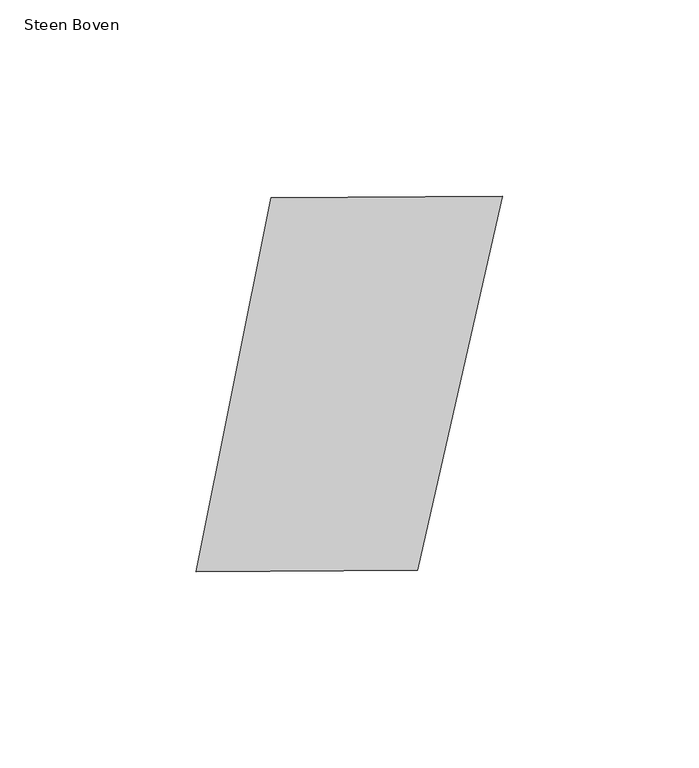
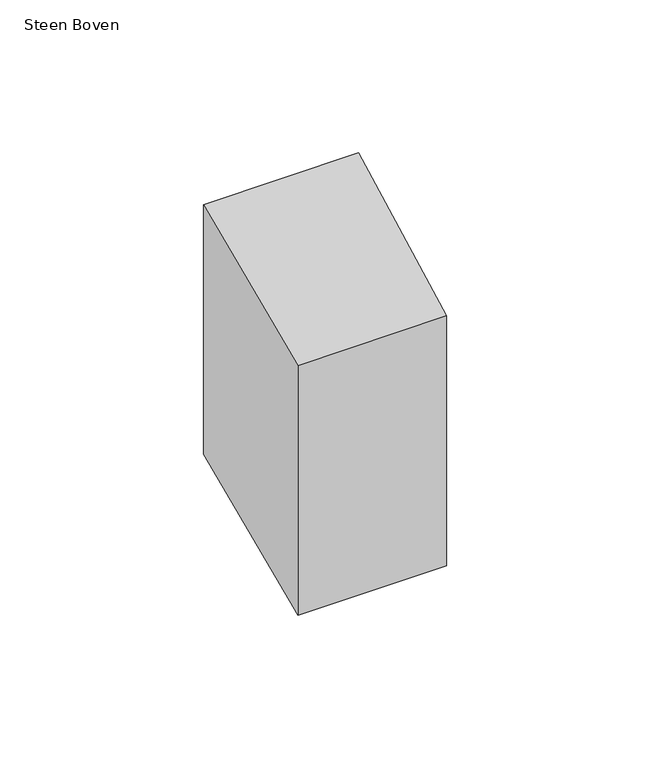
"""IFC4 building model written with IfcOpenShell, lengths in millimetres: proxy geometry, 00_GMA_steen_versie_4 : Steen Boven."""

from ifc_helpers import new_model, si_unit, origin, origin_with_axes, place, context, project, spatial, polyline, outline, extrude, source, transform, mapped, element, save


def steen_boven_9bb71775(model_context):
    return source(origin(), model_context, "Body", "SweptSolid", [
        extrude(outline(polyline([(111.9849233, 118.6347443), (90.2344792, 23.3760955), (33.8999775, 23.0709028), (53.0204132, 118.2901143), (111.9849233, 118.6347443)])), origin_with_axes(), (0.0, 0.0, 1.0), 100.0),
    ])


if __name__ == "__main__":
    model = new_model("IFC4")
    model_context = context("Model", 3, world=origin())
    ifc_project = project(units=[si_unit("LENGTHUNIT", "METRE", prefix="MILLI")], contexts=[model_context])
    site = spatial("IfcSite", under=ifc_project)
    building = spatial("IfcBuilding", under=site)
    placement = place(None, origin())
    steen_boven_shape = steen_boven_9bb71775(model_context)
    element("IfcBuildingElementProxy", 1, Name="00_GMA_steen_versie_4 : Steen Boven", ObjectType="00_GMA_steen_versie_4 : Steen Boven", at=placement, inside=building, context=model_context, shape_type="MappedRepresentation", body=[
        mapped(steen_boven_shape, transform((0.0, 0.0, 0.0), x_axis=(1.0, 0.0, 0.0), y_axis=(0.0, 1.0, 0.0), z_axis=(0.0, 0.0, 1.0))),
    ])
    save(model, "model.ifc")

# Revit data of these elements
# Type "00_GMA_steen_versie_4 : Steen Boven"
#   StootVoegHalfBoven [instance default] = 5 mm
#   StootVoegHalf [instance default] = 5 mm
#   StootVoegBreedteOnder = 10 mm
#   StootVoegBreedteBoven = 10 mm
#   Steendikte = 100 mm
#   LintVoegOnderHalf = 5 mm
#   LintVoegOnder = 10 mm
#   LintVoegBovenHalf = 0 mm
#   LintVoegBoven = 0 mm
#   materiaal = none
#   MateriaalVoeg = none
#   Default Elevation = 0
